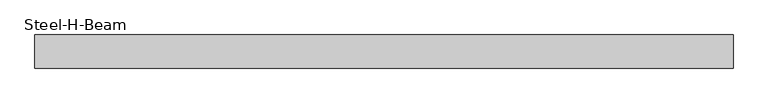
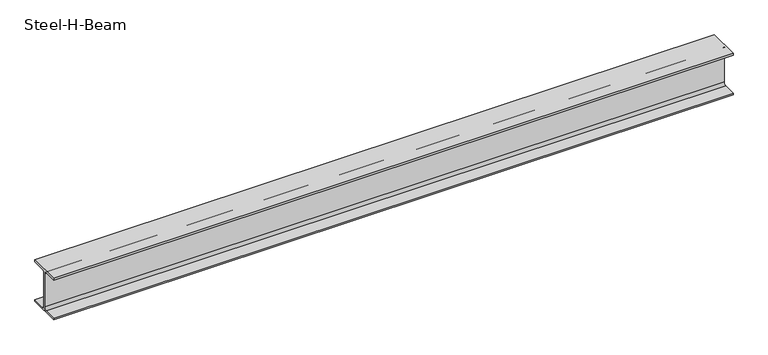
"""IFC4 building model written with IfcOpenShell, lengths in millimetres: beam geometry, Steel-H-Beam : BM121_H-340×250x9x14."""

from ifc_helpers import new_model, si_unit, point, frame, frame_2d, origin, place, context, project, spatial, polyline, circle_curve, trimmed, segment, composite_curve, outline, extrude, source, transform, mapped, element, save


def steel_h_beam_04323a77(model_context):
    return source(origin(), model_context, "Body", "SweptSolid", [
        extrude(outline(composite_curve([segment(polyline([(125.0, -156.0), (125.0, -170.0), (-125.0, -170.0), (-125.0, -156.0), (-24.5, -156.0)]), True, "CONTINUOUS"), segment(trimmed(circle_curve(frame_2d((-24.5, -136.0)), 20.0), [point((-24.5, -156.0))], [point((-4.5, -136.0))], True, "CARTESIAN"), True, "CONTINUOUS"), segment(polyline([(-4.5, -136.0), (-4.5, 136.0)]), True, "CONTINUOUS"), segment(trimmed(circle_curve(frame_2d((-24.5, 136.0)), 20.0), [point((-4.5, 136.0))], [point((-24.5, 156.0))], True, "CARTESIAN"), True, "CONTINUOUS"), segment(polyline([(-24.5, 156.0), (-125.0, 156.0), (-125.0, 170.0), (125.0, 170.0), (125.0, 156.0), (24.5, 156.0)]), True, "CONTINUOUS"), segment(trimmed(circle_curve(frame_2d((24.5, 136.0)), 20.0), [point((24.5, 156.0))], [point((4.5, 136.0))], True, "CARTESIAN"), True, "CONTINUOUS"), segment(polyline([(4.5, 136.0), (4.5, -136.0)]), True, "CONTINUOUS"), segment(trimmed(circle_curve(frame_2d((24.5, -136.0)), 20.0), [point((4.5, -136.0))], [point((24.5, -156.0))], True, "CARTESIAN"), True, "CONTINUOUS"), segment(polyline([(24.5, -156.0), (125.0, -156.0)]), True, "CONTINUOUS")], self_intersect=False)), frame((-2524.0357919, 0.0, 0.0), z_axis=(1.0, 0.0, 0.0), x_axis=(0.0, 1.0, 0.0)), (0.0, 0.0, 1.0), 5262.1606688),
    ])


if __name__ == "__main__":
    model = new_model("IFC4")
    model_context = context("Model", 3, world=origin())
    ifc_project = project(units=[si_unit("LENGTHUNIT", "METRE", prefix="MILLI")], contexts=[model_context])
    site = spatial("IfcSite", under=ifc_project)
    building = spatial("IfcBuilding", under=site)
    placement = place(None, origin())
    steel_h_beam_shape = steel_h_beam_04323a77(model_context)
    element("IfcBeam", 1, ObjectType="Steel-H-Beam : BM121_H-340×250x9x14", at=placement, inside=building, context=model_context, shape_type="MappedRepresentation", body=[
        mapped(steel_h_beam_shape, transform((0.0, 0.0, 0.0), x_axis=(1.0, 0.0, 0.0), y_axis=(0.0, 1.0, 0.0), z_axis=(0.0, 0.0, 1.0))),
    ])
    save(model, "model.ifc")

# Revit data of these elements
# Type "Steel-H-Beam : BM121_H-340×250x9x14"
#   Surface Area = 1.62766 m²/m
#   Section Area = 101.514 cm²
#   Mass per Unit Length = 79.6882 kg/m
#   Length [instance default] = 3000 mm
#   B = 250 mm
#   H = 340 mm
#   r = 20 mm
#   tw = 9 mm
#   tf = 14 mm
#   hec_material4 [instance default] = none
#   hec_material3 [instance default] = none
#   hec_material2 [instance default] = none
#   hec_material1 [instance default] = none
#   Structural Material [instance default] = Steel, 45-345
#   Assembly Code = ""
# Element 1 (IfcBeam, "Steel-H-Beam : BM121_H-340×250x9x14")
#   hec_material4 = S01AA010-00002_Main Steel Structure Fabrication Work_Shelter/Building_Steel Painting/Coating_for Fireproofed Steel Surface, Surface Preparation & Primer Coat
#   hec_material3 = F01AC000-00002_Building/Shelter Fire Proofing Work_Intumescent Coating Type_1 hr. rating (UL 1709))
#   hec_material2 = S01AA010-00002_Main Steel Structure Fabrication Work_Shelter/Building_Steel Painting/Coating_for Fireproofed Steel Surface, Surface Preparation & Primer Coat
#   hec_material1 = S03AA028-00001_Main Steel Structure Erection Work_Shelter/Building_Medium Steel
#   Structural Material = S01AA002-00001_Main Steel Structure Fabrication Work_Shelter/Building_Medium Steel - Standard
#   Materials on its faces: "S01AA002-00001_Main Steel Structure Fabrication Work_Shelter/Building_Medium Steel - Standard"
# Materials
#   "Steel, 45-345": class "Metal", colour RGB 189 187 185, transparency 0, Description = "Steel 345 MPa", Cost = 0
#   "S01AA002-00001_Main Steel Structure Fabrication Work_Shelter/Building_Medium Steel - Standard": class "Metal", colour RGB 120 120 120, transparency 0, Comments = "(90KG/M>Weight≥30KG/M)", Description = "Structural steel 50ksi", W00) Work Master Code = "S01AA002-0001", W01) Work Master_Lv1 = "Main Steel Structure Fabrication Work", W02) Work Master_Lv2 = "Shelter/Building", W03) Work Master_Spec.1 = "Medium Steel - Standard (90KG/M>Weight≥30KG/M)", Cost = 0
#   "S01AA010-00002_Main Steel Structure Fabrication Work_Shelter/Building_Steel Painting/Coating_for Fireproofed Steel Surface, Surface Preparation & Primer Coat": class "Metal", colour RGB 120 120 120, transparency 0, Description = "Paint finished steel", W00) Work Master Code = "SS01AA010-00002", W01) Work Master_Lv1 = "Main Steel Structure Fabrication Work", W02) Work Master_Lv2 = "Shelter/Building", W03) Work Master_Spec.1 = "Steel Painting/Coating", W04) Work Master_Spec.2 = "for Fireproofed Steel Surface, Surface Preparation & Primer Coat", Cost = 0
#   "F01AC000-00002_Building/Shelter Fire Proofing Work_Intumescent Coating Type_1 hr. rating (UL 1709))": class "Metal", colour RGB 255 128 128, transparency 0, Description = "Paint finished steel", W00) Work Master Code = "F01AC000-00002", W01) Work Master_Lv1 = "Building/Shelter Fire Proofing Work", W02) Work Master_Lv2 = "Intumescent Coating Type", W03) Work Master_Spec.1 = "1 hr. rating (UL 1709)", Cost = 0
#   "S03AA028-00001_Main Steel Structure Erection Work_Shelter/Building_Medium Steel": class "Metal", colour RGB 120 120 120, transparency 0, Comments = "(90KG/M>Weight≥30KG/M)", Description = "Structural steel 50ksi", W00) Work Master Code = "S03AA028-0001", W01) Work Master_Lv1 = "Main Steel Structure Erection Work", W02) Work Master_Lv2 = "Shelter/Building", W03) Work Master_Spec.1 = "Medium Steel (90KG/M>Weight≥30KG/M)", Cost = 0
